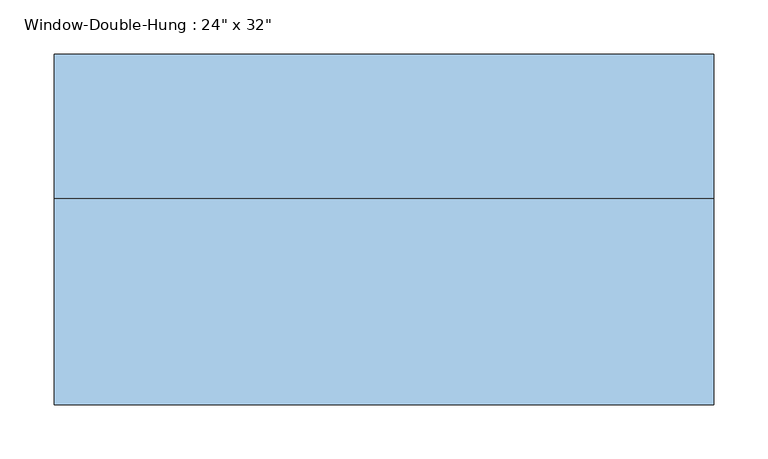
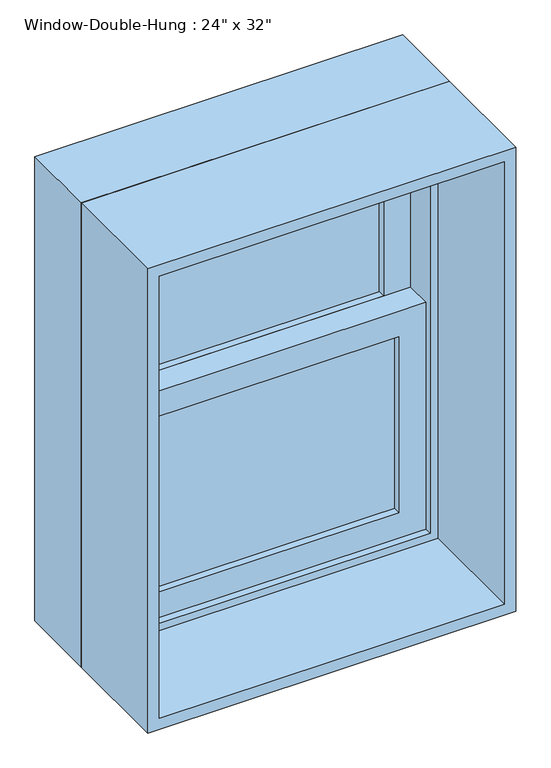
"""IFC4 building model written with IfcOpenShell, lengths in millimetres: window geometry."""

from ifc_helpers import new_model, si_unit, frame, origin, place, context, project, spatial, polyline, outline, extrude, source, transform, mapped, element, save


def window_691d4967(model_context):
    return source(origin(), model_context, "Body", "SweptSolid", [
        extrude(outline(polyline([(228.6, 82.55), (228.6, 76.2), (-228.6, 76.2), (-228.6, 82.55), (228.6, 82.55)])), frame((0.0, 0.0, 990.6), z_axis=(0.0, 0.0, 1.0), x_axis=(1.0, 0.0, 0.0)), (0.0, 0.0, 1.0), 307.975),
        extrude(outline(polyline([(-228.6, 69.85), (228.6, 69.85), (228.6, 63.5), (-228.6, 63.5), (-228.6, 69.85)])), frame((0.0, 0.0, 990.6), z_axis=(0.0, 0.0, 1.0), x_axis=(1.0, 0.0, 0.0)), (0.0, 0.0, 1.0), 307.975),
        extrude(outline(polyline([(228.6, 127.0), (228.6, 120.65), (-228.6, 120.65), (-228.6, 127.0), (228.6, 127.0)])), frame((0.0, 0.0, 1343.025), z_axis=(0.0, 0.0, 1.0), x_axis=(1.0, 0.0, 0.0)), (0.0, 0.0, 1.0), 307.975),
        extrude(outline(polyline([(-228.6, 114.3), (228.6, 114.3), (228.6, 107.95), (-228.6, 107.95), (-228.6, 114.3)])), frame((0.0, 0.0, 1343.025), z_axis=(0.0, 0.0, 1.0), x_axis=(1.0, 0.0, 0.0)), (0.0, 0.0, 1.0), 307.975),
        extrude(outline(polyline([(1343.025, -273.05), (946.15, -273.05), (946.15, 273.05), (1343.025, 273.05), (1343.025, -273.05)]), holes=[polyline([(1298.575, 228.6), (990.6, 228.6), (990.6, -228.6), (1298.575, -228.6), (1298.575, 228.6)])]), frame((0.0, 50.8, 0.0), z_axis=(0.0, 1.0, 0.0), x_axis=(0.0, 0.0, 1.0)), (0.0, 0.0, 1.0), 44.45),
        extrude(outline(polyline([(1695.45, -273.05), (1298.575, -273.05), (1298.575, 273.05), (1695.45, 273.05), (1695.45, -273.05)]), holes=[polyline([(1651.0, 228.6), (1343.025, 228.6), (1343.025, -228.6), (1651.0, -228.6), (1651.0, 228.6)])]), frame((0.0, 95.25, 0.0), z_axis=(0.0, 1.0, 0.0), x_axis=(0.0, 0.0, 1.0)), (0.0, 0.0, 1.0), 44.45),
        extrude(outline(polyline([(1727.2, -304.8), (914.4, -304.8), (914.4, 304.8), (1727.2, 304.8), (1727.2, -304.8)]), holes=[polyline([(1695.45, 273.05), (946.15, 273.05), (946.15, -273.05), (1695.45, -273.05), (1695.45, 273.05)])]), frame((0.0, 38.1, 0.0), z_axis=(0.0, 1.0, 0.0), x_axis=(0.0, 0.0, 1.0)), (0.0, 0.0, 1.0), 133.35),
        extrude(outline(polyline([(1727.2, 304.8), (1727.2, -304.8), (914.4, -304.8), (914.4, 304.8), (1727.2, 304.8)]), holes=[polyline([(1708.15, 285.75), (933.45, 285.75), (933.45, -285.75), (1708.15, -285.75), (1708.15, 285.75)])]), frame((0.0, -152.4, 0.0), z_axis=(0.0, 1.0, 0.0), x_axis=(0.0, 0.0, 1.0)), (0.0, 0.0, 1.0), 190.5),
    ])


if __name__ == "__main__":
    model = new_model("IFC4")
    model_context = context("Model", 3, world=origin())
    ifc_project = project(units=[si_unit("LENGTHUNIT", "METRE", prefix="MILLI")], contexts=[model_context])
    site = spatial("IfcSite", under=ifc_project)
    building = spatial("IfcBuilding", under=site)
    placement = place(None, origin())
    window_shape = window_691d4967(model_context)
    element("IfcWindow", 1, ObjectType="Window-Double-Hung : 24\" x 32\"", at=placement, inside=building, context=model_context, shape_type="MappedRepresentation", body=[
        mapped(window_shape, transform((0.0, 0.0, 0.0), x_axis=(1.0, 0.0, 0.0), y_axis=(0.0, 1.0, 0.0), z_axis=(0.0, 0.0, 1.0))),
    ])
    save(model, "model.ifc")

# Revit data of these elements
# Type "Window-Double-Hung : 24\" x 32\""
#   Type Mark = "20"
#   Fire Rating = "0.5h"
#   Construction Type Id = "DG-DR"
#   Assembly Code = "B2020100"
#   Analytic Construction = "Double glazing - domestic"
#   Wall Thickness [instance default] = 0' - 6"
#   Window Inset [instance default] = 0' - 0"
#   Visual Light Transmittance = 0.81
#   Thermal Resistance (R) = 1.8146 (h·ft²·°F)/BTU
#   Solar Heat Gain Coefficient = 0.76
#   Muntin Width = 1' - 6"
#   Muntin Height = 1' - 0 1/8"
#   Interior Wall Closure [instance default] = 0' - 1 1/2"
#   Rough Width = 2' - 0 1/2"
#   Rough Height = 2' - 8 1/2"
#   Frame Extension [instance default] = 0' - 1 1/4"
#   Exterior Wall Closure [instance default] = 0' - 0 1/2"
#   Extension Jamb [instance default] = 0' - 1 1/2"
#   Heat Transfer Coefficient (U) = 0.5511 BTU/(h·ft²·°F)
#   Height = 2' - 8"
#   Width = 2' - 0"
#   Top Muntin Visibility = yes
#   Indicator Visibility [instance default] = yes
#   Extension Jamb Visibility [instance default] = yes
#   Interior Trim Visibility [instance default] = yes
#   Exterior Trim Visibility [instance default] = yes
#   Define Thermal Properties by = 1
#   Bottom Muntin Visibility = yes
#   Muntin Pattern = Muntin Pattern_2x2 : Muntin Pattern_2x2
#   Interior Trim Material = Wood - Stained
#   Interior Trim = Trim-Window-Interior-Flat : Picture Frame
#   Exterior Trim Material = Clad - White
#   Exterior Trim = Trim-Window-Exterior-Flat : with Sill
#   Glass Panel Material = Glass
#   Exterior Frame Material = Clad - White
#   Interior Frame Material = Wood - Stained
#   Wall Closure = (empty or 0)
# Element 1 (IfcWindow, "Window-Double-Hung : 24\" x 32\"")
#   Wall Thickness = 1' - 0"
#   Extension Jamb = 0' - 7 1/2"
#   Materials on its faces: "Wood - Stained", "Glass", "Clad - White"
# Materials
#   "Wood - Stained": class "Wood", colour RGB 224 178 126, transparency 0, Cost = 0
#   "Clad - White": class "Wood", colour RGB 242 242 238, transparency 0, Cost = 0
#   "Glass": class "Glass", colour RGB 0 128 192, transparency 0.75, Description = "Soda Lime Glass", Cost = 0
